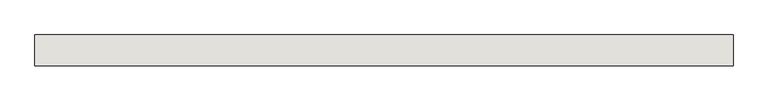
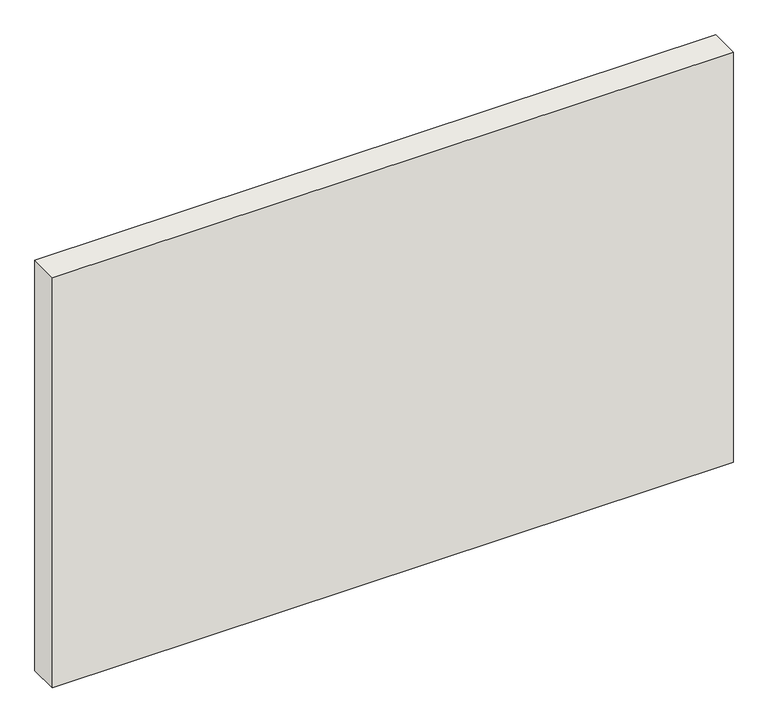
"""IFC4 building model written with IfcOpenShell, lengths in millimetres: wall geometry, Holzwand."""

from ifc_helpers import new_model, si_unit, origin, origin_with_axes, place, context, project, spatial, polyline, outline, extrude, source, transform, mapped, element, save


def wall_5eab4a6d(model_context):
    return source(origin(), model_context, "Body", "SweptSolid", [
        extrude(outline(polyline([(4520.0, 200.0), (4520.0, 0.0), (0.0, 0.0), (0.0, 200.0), (4520.0, 200.0)])), origin_with_axes(), (0.0, 0.0, 1.0), 2880.0),
    ])


if __name__ == "__main__":
    model = new_model("IFC4")
    model_context = context("Model", 3, world=origin())
    ifc_project = project(units=[si_unit("LENGTHUNIT", "METRE", prefix="MILLI")], contexts=[model_context])
    site = spatial("IfcSite", under=ifc_project)
    building = spatial("IfcBuilding", under=site)
    placement = place(None, origin())
    wall_shape = wall_5eab4a6d(model_context)
    element("IfcWall", 1, ObjectType="Holzwand", at=placement, inside=building, context=model_context, shape_type="MappedRepresentation", body=[
        mapped(wall_shape, transform((0.0, 0.0, 0.0), x_axis=(1.0, 0.0, 0.0), y_axis=(0.0, 1.0, 0.0), z_axis=(0.0, 0.0, 1.0))),
    ])
    save(model, "model.ifc")

# Revit data of these elements
# Element 1 (IfcWall, "Holzwand")
#   Materials on its faces: "holzschalung"
# Materials
#   "holzschalung": class "Unassigned", colour RGB 128 128 128, transparency 0
